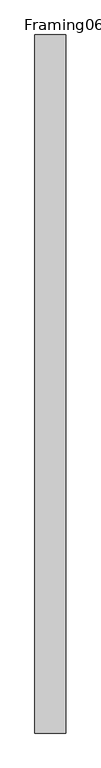
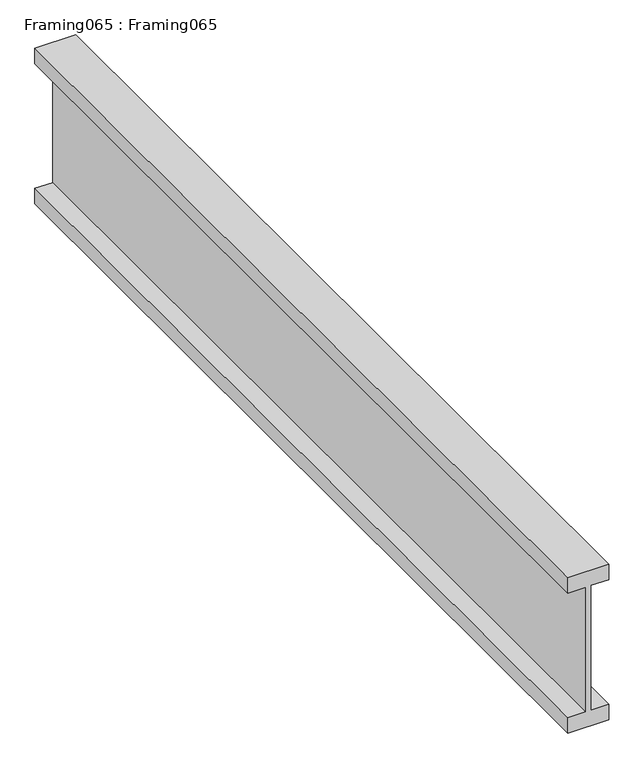
"""IFC4 building model written with IfcOpenShell, lengths in millimetres: proxy geometry, Framing065 : Framing065."""

from ifc_helpers import new_model, si_unit, frame, origin, place, context, project, spatial, polyline, outline, extrude, source, transform, mapped, element, save


def framing065_framing065_252a1c86(model_context):
    return source(origin(), model_context, "Body", "SweptSolid", [
        extrude(outline(polyline([(40077.771, 8096.295938), (39792.021, 8096.295938), (39792.021, 8057.402188), (39757.096, 8057.402188), (39757.096, 8146.302188), (39792.021, 8146.302188), (39792.021, 8107.408438), (40077.771, 8107.408438), (40077.771, 8146.302188), (40112.696, 8146.302188), (40112.696, 8057.402188), (40077.771, 8057.402188), (40077.771, 8096.295938)])), frame((0.0, -3747.9491938, 0.0), z_axis=(0.0, 1.0, 0.0), x_axis=(0.0, 0.0, 1.0)), (0.0, 0.0, 1.0), 2000.0),
    ])


if __name__ == "__main__":
    model = new_model("IFC4")
    model_context = context("Model", 3, world=origin())
    ifc_project = project(units=[si_unit("LENGTHUNIT", "METRE", prefix="MILLI")], contexts=[model_context])
    site = spatial("IfcSite", under=ifc_project)
    building = spatial("IfcBuilding", under=site)
    placement = place(None, origin())
    framing065_framing065_shape = framing065_framing065_252a1c86(model_context)
    element("IfcBuildingElementProxy", 1, Name="Framing065 : Framing065", ObjectType="Framing065 : Framing065", at=placement, inside=building, context=model_context, shape_type="MappedRepresentation", body=[
        mapped(framing065_framing065_shape, transform((0.0, 0.0, 0.0), x_axis=(1.0, 0.0, 0.0), y_axis=(0.0, 1.0, 0.0), z_axis=(0.0, 0.0, 1.0))),
    ])
    save(model, "model.ifc")

# Revit data of these elements
# Type "Framing065 : Framing065"
#   NameOverride = "Framing065"
# Element 1 (IfcBuildingElementProxy, "Framing065 : Framing065")
#   Materials on its faces: "WOOD FRAMING (SEE STRUCT DWGS)"
# Materials
#   "WOOD FRAMING (SEE STRUCT DWGS)": class "Unassigned", colour RGB 224 188 168, transparency 0, Cost = 0
